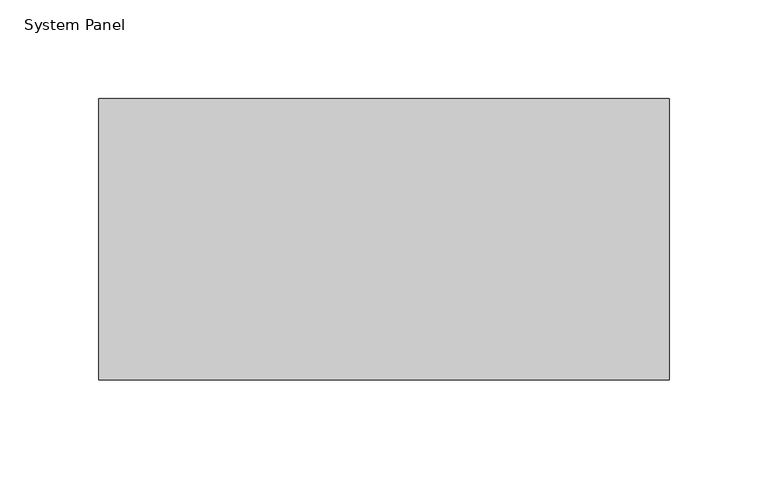
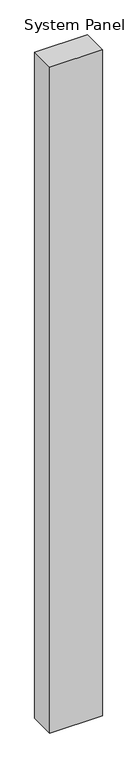
"""IFC4 building model written with IfcOpenShell, lengths in millimetres: plate geometry, System Panel : NLRS_21_CWP_hsb-vulling minerale wol 142 _gen_rsf."""

from ifc_helpers import new_model, si_unit, origin, origin_with_axes, place, context, project, spatial, polyline, outline, extrude, source, transform, mapped, element, save


def system_panel_3da1e079(model_context):
    return source(origin(), model_context, "Body", "SweptSolid", [
        extrude(outline(polyline([(144.0000002, -71.0), (-144.0000002, -71.0), (-144.0000002, 71.0), (144.0000002, 71.0), (144.0000002, -71.0)])), origin_with_axes(), (0.0, 0.0, 1.0), 3849.0),
    ])


if __name__ == "__main__":
    model = new_model("IFC4")
    model_context = context("Model", 3, world=origin())
    ifc_project = project(units=[si_unit("LENGTHUNIT", "METRE", prefix="MILLI")], contexts=[model_context])
    site = spatial("IfcSite", under=ifc_project)
    building = spatial("IfcBuilding", under=site)
    placement = place(None, origin())
    system_panel_shape = system_panel_3da1e079(model_context)
    element("IfcPlate", 1, ObjectType="System Panel : NLRS_21_CWP_hsb-vulling minerale wol 142 _gen_rsf", at=placement, inside=building, context=model_context, shape_type="MappedRepresentation", body=[
        mapped(system_panel_shape, transform((0.0, 0.0, 0.0), x_axis=(1.0, 0.0, 0.0), y_axis=(0.0, 1.0, 0.0), z_axis=(0.0, 0.0, 1.0))),
    ])
    save(model, "model.ifc")

# Revit data of these elements
# Type "System Panel : NLRS_21_CWP_hsb-vulling minerale wol 142 _gen_rsf"
#   Export Type to IFC As = "IfcWall"
#   Type IfcGUID = "07M7mRoiH1CR8m_RSKIwpC"
#   Assembly Code = "21.23"
# Element 1 (IfcPlate, "System Panel : NLRS_21_CWP_hsb-vulling minerale wol 142 _gen_rsf")
#   Materials on its faces: "NLRS_m1_isolatie minerale wol_gen_rsf"
# Materials
#   "NLRS_m1_isolatie minerale wol_gen_rsf": class "M - Anorganische materialen", colour RGB 200 200 140, transparency 0, Keynote = "m1", Manufacturer = "Revit Standards Foundation", URL = "www.revitstandards.org", Description = "isolatie minerale wol", Cost = 0
